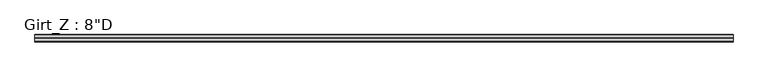
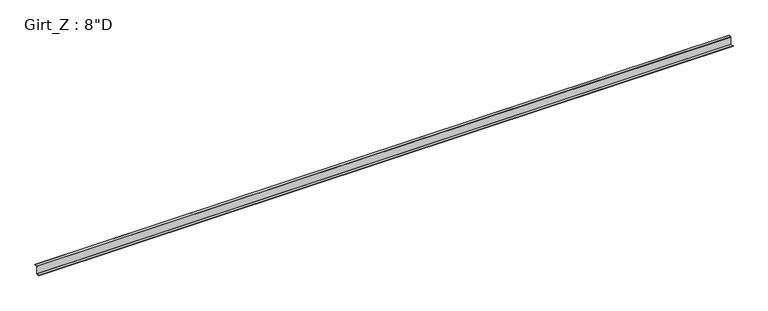
"""IFC4 building model written with IfcOpenShell, lengths in millimetres: beam geometry."""

from ifc_helpers import new_model, si_unit, point, frame, frame_2d, origin, place, context, project, spatial, polyline, circle_curve, trimmed, segment, composite_curve, outline, extrude, source, transform, mapped, element, save


def beam_fc307d6a(model_context):
    return source(origin(), model_context, "Body", "SweptSolid", [
        extrude(outline(composite_curve([segment(polyline([(77.9859375, 101.6), (90.2310415, 87.0068534), (88.1028742, 85.221109), (76.6904765, 98.821875), (3.3005807, 98.821875)]), True, "CONTINUOUS"), segment(trimmed(circle_curve(frame_2d((3.3741066, 96.8381931)), 1.9850441), [point((3.3005807, 98.821875))], [point((1.3890625, 96.8381931))], True, "CARTESIAN"), True, "CONTINUOUS"), segment(polyline([(1.3890625, 96.8381931), (1.3890625, -101.6), (-84.3359375, -101.6), (-96.5810415, -87.0068534), (-94.4528742, -85.221109), (-83.0404765, -98.821875), (-3.2694106, -98.821875)]), True, "CONTINUOUS"), segment(trimmed(circle_curve(frame_2d((-3.3748024, -96.8389339)), 1.9857399), [point((-3.2694106, -98.821875))], [point((-1.3890625, -96.8389339))], True, "CARTESIAN"), True, "CONTINUOUS"), segment(polyline([(-1.3890625, -96.8389339), (-1.3890625, 96.8375)]), True, "CONTINUOUS"), segment(trimmed(circle_curve(frame_2d((3.3734375, 96.8375)), 4.7625), [point((-1.3890625, 96.8375))], [point((3.3734375, 101.6))], False, "CARTESIAN"), True, "CONTINUOUS"), segment(polyline([(3.3734375, 101.6), (77.9859375, 101.6)]), True, "CONTINUOUS")], self_intersect=False)), frame((-9004.696875, 0.0, 0.0), z_axis=(1.0, 0.0, 0.0), x_axis=(0.0, 1.0, 0.0)), (0.0, 0.0, 1.0), 17843.5),
    ])


if __name__ == "__main__":
    model = new_model("IFC4")
    model_context = context("Model", 3, world=origin())
    ifc_project = project(units=[si_unit("LENGTHUNIT", "METRE", prefix="MILLI")], contexts=[model_context])
    site = spatial("IfcSite", under=ifc_project)
    building = spatial("IfcBuilding", under=site)
    placement = place(None, origin())
    beam_shape = beam_fc307d6a(model_context)
    element("IfcBeam", 1, ObjectType="Girt_Z : 8\"D", at=placement, inside=building, context=model_context, shape_type="MappedRepresentation", body=[
        mapped(beam_shape, transform((0.0, 0.0, 0.0), x_axis=(1.0, 0.0, 0.0), y_axis=(0.0, 1.0, 0.0), z_axis=(0.0, 0.0, 1.0))),
    ])
    save(model, "model.ifc")

# Revit data of these elements
# Type "Girt_Z : 8\"D"
#   half leg = 0' - 1 11/16"
#   Web_Thickness = 0' - 0 7/64"
#   Length [instance default] = 10' - 0"
#   Leg_2 = 0' - 3 3/8"
#   Leg_1 = 0' - 3 1/8"
#   Height = 0' - 8"
#   Structural Material [instance default] = none
